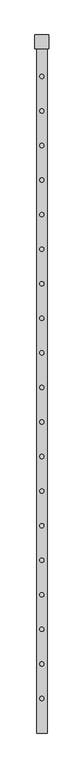
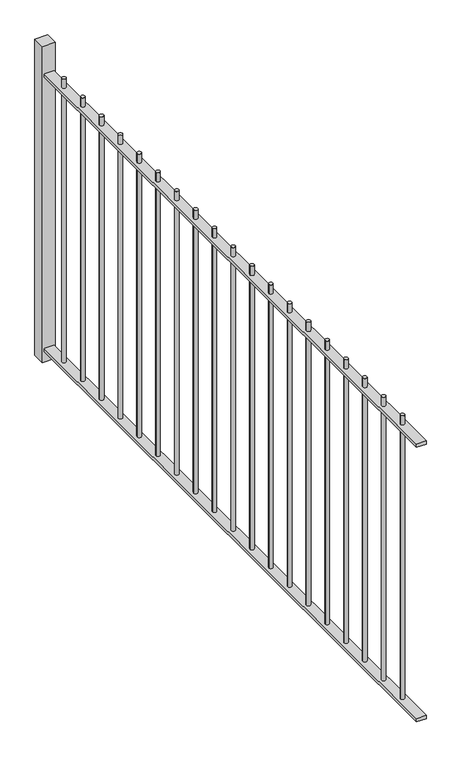
"""IFC4 building model written with IfcOpenShell, lengths in millimetres: railing geometry."""

from ifc_helpers import new_model, si_unit, point, frame, frame_2d, origin, place, context, project, spatial, polyline, circle_curve, trimmed, segment, composite_curve, outline, extrude, source, transform, mapped, element, save


def railing_16b95b7e(model_context):
    return source(origin(), model_context, "Body", "SweptSolid", [
        extrude(outline(polyline([(-6549.419961, -12811.1119119), (-6489.419961, -12811.1119119), (-6489.419961, -16811.1119119), (-6549.419961, -16811.1119119), (-6549.419961, -12811.1119119)])), frame((0.0, 0.0, -30.0), z_axis=(0.0, 0.0, 1.0), x_axis=(1.0, 0.0, 0.0)), (0.0, 0.0, 1.0), 20.0),
        extrude(outline(polyline([(-6549.419961, -12811.1119119), (-6489.419961, -12811.1119119), (-6489.419961, -16811.1119119), (-6549.419961, -16811.1119119), (-6549.419961, -12811.1119119)])), frame((0.0, 0.0, 1750.0), z_axis=(0.0, 0.0, 1.0), x_axis=(1.0, 0.0, 0.0)), (0.0, 0.0, 1.0), 20.0),
        extrude(outline(composite_curve([segment(trimmed(circle_curve(frame_2d((-6519.419961, -16611.1119119)), 12.5), [point((-6531.919961, -16611.1119119))], [point((-6506.919961, -16611.1119119))], False, "CARTESIAN"), True, "CONTINUOUS"), segment(trimmed(circle_curve(frame_2d((-6519.419961, -16611.1119119)), 12.5), [point((-6506.919961, -16611.1119119))], [point((-6531.919961, -16611.1119119))], False, "CARTESIAN"), True, "CONTINUOUS")], self_intersect=False)), frame((0.0, 0.0, -10.0), z_axis=(0.0, 0.0, 1.0), x_axis=(1.0, 0.0, 0.0)), (0.0, 0.0, 1.0), 1840.0),
        extrude(outline(composite_curve([segment(trimmed(circle_curve(frame_2d((-6519.419961, -16411.1119119)), 12.5), [point((-6531.919961, -16411.1119119))], [point((-6506.919961, -16411.1119119))], False, "CARTESIAN"), True, "CONTINUOUS"), segment(trimmed(circle_curve(frame_2d((-6519.419961, -16411.1119119)), 12.5), [point((-6506.919961, -16411.1119119))], [point((-6531.919961, -16411.1119119))], False, "CARTESIAN"), True, "CONTINUOUS")], self_intersect=False)), frame((0.0, 0.0, -10.0), z_axis=(0.0, 0.0, 1.0), x_axis=(1.0, 0.0, 0.0)), (0.0, 0.0, 1.0), 1840.0),
        extrude(outline(composite_curve([segment(trimmed(circle_curve(frame_2d((-6519.419961, -16211.1119119)), 12.5), [point((-6531.919961, -16211.1119119))], [point((-6506.919961, -16211.1119119))], False, "CARTESIAN"), True, "CONTINUOUS"), segment(trimmed(circle_curve(frame_2d((-6519.419961, -16211.1119119)), 12.5), [point((-6506.919961, -16211.1119119))], [point((-6531.919961, -16211.1119119))], False, "CARTESIAN"), True, "CONTINUOUS")], self_intersect=False)), frame((0.0, 0.0, -10.0), z_axis=(0.0, 0.0, 1.0), x_axis=(1.0, 0.0, 0.0)), (0.0, 0.0, 1.0), 1840.0),
        extrude(outline(composite_curve([segment(trimmed(circle_curve(frame_2d((-6519.419961, -16011.1119119)), 12.5), [point((-6531.919961, -16011.1119119))], [point((-6506.919961, -16011.1119119))], False, "CARTESIAN"), True, "CONTINUOUS"), segment(trimmed(circle_curve(frame_2d((-6519.419961, -16011.1119119)), 12.5), [point((-6506.919961, -16011.1119119))], [point((-6531.919961, -16011.1119119))], False, "CARTESIAN"), True, "CONTINUOUS")], self_intersect=False)), frame((0.0, 0.0, -10.0), z_axis=(0.0, 0.0, 1.0), x_axis=(1.0, 0.0, 0.0)), (0.0, 0.0, 1.0), 1840.0),
        extrude(outline(composite_curve([segment(trimmed(circle_curve(frame_2d((-6519.419961, -15811.1119119)), 12.5), [point((-6531.919961, -15811.1119119))], [point((-6506.919961, -15811.1119119))], False, "CARTESIAN"), True, "CONTINUOUS"), segment(trimmed(circle_curve(frame_2d((-6519.419961, -15811.1119119)), 12.5), [point((-6506.919961, -15811.1119119))], [point((-6531.919961, -15811.1119119))], False, "CARTESIAN"), True, "CONTINUOUS")], self_intersect=False)), frame((0.0, 0.0, -10.0), z_axis=(0.0, 0.0, 1.0), x_axis=(1.0, 0.0, 0.0)), (0.0, 0.0, 1.0), 1840.0),
        extrude(outline(composite_curve([segment(trimmed(circle_curve(frame_2d((-6519.419961, -15611.1119119)), 12.5), [point((-6531.919961, -15611.1119119))], [point((-6506.919961, -15611.1119119))], False, "CARTESIAN"), True, "CONTINUOUS"), segment(trimmed(circle_curve(frame_2d((-6519.419961, -15611.1119119)), 12.5), [point((-6506.919961, -15611.1119119))], [point((-6531.919961, -15611.1119119))], False, "CARTESIAN"), True, "CONTINUOUS")], self_intersect=False)), frame((0.0, 0.0, -10.0), z_axis=(0.0, 0.0, 1.0), x_axis=(1.0, 0.0, 0.0)), (0.0, 0.0, 1.0), 1840.0),
        extrude(outline(composite_curve([segment(trimmed(circle_curve(frame_2d((-6519.419961, -15411.1119119)), 12.5), [point((-6531.919961, -15411.1119119))], [point((-6506.919961, -15411.1119119))], False, "CARTESIAN"), True, "CONTINUOUS"), segment(trimmed(circle_curve(frame_2d((-6519.419961, -15411.1119119)), 12.5), [point((-6506.919961, -15411.1119119))], [point((-6531.919961, -15411.1119119))], False, "CARTESIAN"), True, "CONTINUOUS")], self_intersect=False)), frame((0.0, 0.0, -10.0), z_axis=(0.0, 0.0, 1.0), x_axis=(1.0, 0.0, 0.0)), (0.0, 0.0, 1.0), 1840.0),
        extrude(outline(composite_curve([segment(trimmed(circle_curve(frame_2d((-6519.419961, -15211.1119119)), 12.5), [point((-6531.919961, -15211.1119119))], [point((-6506.919961, -15211.1119119))], False, "CARTESIAN"), True, "CONTINUOUS"), segment(trimmed(circle_curve(frame_2d((-6519.419961, -15211.1119119)), 12.5), [point((-6506.919961, -15211.1119119))], [point((-6531.919961, -15211.1119119))], False, "CARTESIAN"), True, "CONTINUOUS")], self_intersect=False)), frame((0.0, 0.0, -10.0), z_axis=(0.0, 0.0, 1.0), x_axis=(1.0, 0.0, 0.0)), (0.0, 0.0, 1.0), 1840.0),
        extrude(outline(composite_curve([segment(trimmed(circle_curve(frame_2d((-6519.419961, -15011.1119119)), 12.5), [point((-6531.919961, -15011.1119119))], [point((-6506.919961, -15011.1119119))], False, "CARTESIAN"), True, "CONTINUOUS"), segment(trimmed(circle_curve(frame_2d((-6519.419961, -15011.1119119)), 12.5), [point((-6506.919961, -15011.1119119))], [point((-6531.919961, -15011.1119119))], False, "CARTESIAN"), True, "CONTINUOUS")], self_intersect=False)), frame((0.0, 0.0, -10.0), z_axis=(0.0, 0.0, 1.0), x_axis=(1.0, 0.0, 0.0)), (0.0, 0.0, 1.0), 1840.0),
        extrude(outline(composite_curve([segment(trimmed(circle_curve(frame_2d((-6519.419961, -14811.1119119)), 12.5), [point((-6531.919961, -14811.1119119))], [point((-6506.919961, -14811.1119119))], False, "CARTESIAN"), True, "CONTINUOUS"), segment(trimmed(circle_curve(frame_2d((-6519.419961, -14811.1119119)), 12.5), [point((-6506.919961, -14811.1119119))], [point((-6531.919961, -14811.1119119))], False, "CARTESIAN"), True, "CONTINUOUS")], self_intersect=False)), frame((0.0, 0.0, -10.0), z_axis=(0.0, 0.0, 1.0), x_axis=(1.0, 0.0, 0.0)), (0.0, 0.0, 1.0), 1840.0),
        extrude(outline(composite_curve([segment(trimmed(circle_curve(frame_2d((-6519.419961, -14611.1119119)), 12.5), [point((-6531.919961, -14611.1119119))], [point((-6506.919961, -14611.1119119))], False, "CARTESIAN"), True, "CONTINUOUS"), segment(trimmed(circle_curve(frame_2d((-6519.419961, -14611.1119119)), 12.5), [point((-6506.919961, -14611.1119119))], [point((-6531.919961, -14611.1119119))], False, "CARTESIAN"), True, "CONTINUOUS")], self_intersect=False)), frame((0.0, 0.0, -10.0), z_axis=(0.0, 0.0, 1.0), x_axis=(1.0, 0.0, 0.0)), (0.0, 0.0, 1.0), 1840.0),
        extrude(outline(composite_curve([segment(trimmed(circle_curve(frame_2d((-6519.419961, -14411.1119119)), 12.5), [point((-6531.919961, -14411.1119119))], [point((-6506.919961, -14411.1119119))], False, "CARTESIAN"), True, "CONTINUOUS"), segment(trimmed(circle_curve(frame_2d((-6519.419961, -14411.1119119)), 12.5), [point((-6506.919961, -14411.1119119))], [point((-6531.919961, -14411.1119119))], False, "CARTESIAN"), True, "CONTINUOUS")], self_intersect=False)), frame((0.0, 0.0, -10.0), z_axis=(0.0, 0.0, 1.0), x_axis=(1.0, 0.0, 0.0)), (0.0, 0.0, 1.0), 1840.0),
        extrude(outline(composite_curve([segment(trimmed(circle_curve(frame_2d((-6519.419961, -14211.1119119)), 12.5), [point((-6531.919961, -14211.1119119))], [point((-6506.919961, -14211.1119119))], False, "CARTESIAN"), True, "CONTINUOUS"), segment(trimmed(circle_curve(frame_2d((-6519.419961, -14211.1119119)), 12.5), [point((-6506.919961, -14211.1119119))], [point((-6531.919961, -14211.1119119))], False, "CARTESIAN"), True, "CONTINUOUS")], self_intersect=False)), frame((0.0, 0.0, -10.0), z_axis=(0.0, 0.0, 1.0), x_axis=(1.0, 0.0, 0.0)), (0.0, 0.0, 1.0), 1840.0),
        extrude(outline(composite_curve([segment(trimmed(circle_curve(frame_2d((-6519.419961, -14011.1119119)), 12.5), [point((-6531.919961, -14011.1119119))], [point((-6506.919961, -14011.1119119))], False, "CARTESIAN"), True, "CONTINUOUS"), segment(trimmed(circle_curve(frame_2d((-6519.419961, -14011.1119119)), 12.5), [point((-6506.919961, -14011.1119119))], [point((-6531.919961, -14011.1119119))], False, "CARTESIAN"), True, "CONTINUOUS")], self_intersect=False)), frame((0.0, 0.0, -10.0), z_axis=(0.0, 0.0, 1.0), x_axis=(1.0, 0.0, 0.0)), (0.0, 0.0, 1.0), 1840.0),
        extrude(outline(composite_curve([segment(trimmed(circle_curve(frame_2d((-6519.419961, -13811.1119119)), 12.5), [point((-6531.919961, -13811.1119119))], [point((-6506.919961, -13811.1119119))], False, "CARTESIAN"), True, "CONTINUOUS"), segment(trimmed(circle_curve(frame_2d((-6519.419961, -13811.1119119)), 12.5), [point((-6506.919961, -13811.1119119))], [point((-6531.919961, -13811.1119119))], False, "CARTESIAN"), True, "CONTINUOUS")], self_intersect=False)), frame((0.0, 0.0, -10.0), z_axis=(0.0, 0.0, 1.0), x_axis=(1.0, 0.0, 0.0)), (0.0, 0.0, 1.0), 1840.0),
        extrude(outline(composite_curve([segment(trimmed(circle_curve(frame_2d((-6519.419961, -13611.1119119)), 12.5), [point((-6531.919961, -13611.1119119))], [point((-6506.919961, -13611.1119119))], False, "CARTESIAN"), True, "CONTINUOUS"), segment(trimmed(circle_curve(frame_2d((-6519.419961, -13611.1119119)), 12.5), [point((-6506.919961, -13611.1119119))], [point((-6531.919961, -13611.1119119))], False, "CARTESIAN"), True, "CONTINUOUS")], self_intersect=False)), frame((0.0, 0.0, -10.0), z_axis=(0.0, 0.0, 1.0), x_axis=(1.0, 0.0, 0.0)), (0.0, 0.0, 1.0), 1840.0),
        extrude(outline(composite_curve([segment(trimmed(circle_curve(frame_2d((-6519.419961, -13411.1119119)), 12.5), [point((-6531.919961, -13411.1119119))], [point((-6506.919961, -13411.1119119))], False, "CARTESIAN"), True, "CONTINUOUS"), segment(trimmed(circle_curve(frame_2d((-6519.419961, -13411.1119119)), 12.5), [point((-6506.919961, -13411.1119119))], [point((-6531.919961, -13411.1119119))], False, "CARTESIAN"), True, "CONTINUOUS")], self_intersect=False)), frame((0.0, 0.0, -10.0), z_axis=(0.0, 0.0, 1.0), x_axis=(1.0, 0.0, 0.0)), (0.0, 0.0, 1.0), 1840.0),
        extrude(outline(composite_curve([segment(trimmed(circle_curve(frame_2d((-6519.419961, -13211.1119119)), 12.5), [point((-6531.919961, -13211.1119119))], [point((-6506.919961, -13211.1119119))], False, "CARTESIAN"), True, "CONTINUOUS"), segment(trimmed(circle_curve(frame_2d((-6519.419961, -13211.1119119)), 12.5), [point((-6506.919961, -13211.1119119))], [point((-6531.919961, -13211.1119119))], False, "CARTESIAN"), True, "CONTINUOUS")], self_intersect=False)), frame((0.0, 0.0, -10.0), z_axis=(0.0, 0.0, 1.0), x_axis=(1.0, 0.0, 0.0)), (0.0, 0.0, 1.0), 1840.0),
        extrude(outline(composite_curve([segment(trimmed(circle_curve(frame_2d((-6519.419961, -13011.1119119)), 12.5), [point((-6531.919961, -13011.1119119))], [point((-6506.919961, -13011.1119119))], False, "CARTESIAN"), True, "CONTINUOUS"), segment(trimmed(circle_curve(frame_2d((-6519.419961, -13011.1119119)), 12.5), [point((-6506.919961, -13011.1119119))], [point((-6531.919961, -13011.1119119))], False, "CARTESIAN"), True, "CONTINUOUS")], self_intersect=False)), frame((0.0, 0.0, -10.0), z_axis=(0.0, 0.0, 1.0), x_axis=(1.0, 0.0, 0.0)), (0.0, 0.0, 1.0), 1840.0),
        extrude(outline(polyline([(-6479.419961, -12771.1119119), (-6479.419961, -12851.1119119), (-6559.419961, -12851.1119119), (-6559.419961, -12771.1119119), (-6479.419961, -12771.1119119)])), frame((0.0, 0.0, -100.0), z_axis=(0.0, 0.0, 1.0), x_axis=(1.0, 0.0, 0.0)), (0.0, 0.0, 1.0), 2050.0),
    ])


if __name__ == "__main__":
    model = new_model("IFC4")
    model_context = context("Model", 3, world=origin())
    ifc_project = project(units=[si_unit("LENGTHUNIT", "METRE", prefix="MILLI")], contexts=[model_context])
    site = spatial("IfcSite", under=ifc_project)
    building = spatial("IfcBuilding", under=site)
    placement = place(None, origin())
    railing_shape = railing_16b95b7e(model_context)
    element("IfcRailing", 1, at=placement, inside=building, context=model_context, shape_type="MappedRepresentation", body=[
        mapped(railing_shape, transform((0.0, 0.0, 0.0), x_axis=(1.0, 0.0, 0.0), y_axis=(0.0, 1.0, 0.0), z_axis=(0.0, 0.0, 1.0))),
    ])
    save(model, "model.ifc")

# Revit data of these elements
# Element 1 (IfcRailing)
#   Materials on its faces: "NLRS_h2_staal_generiek zwart_gen_rsf", "NLRS_h2_staal_gen_rsf"
# Materials
#   "NLRS_h2_staal_generiek zwart_gen_rsf": class "Metal", colour RGB 189 187 185, transparency 0, Manufacturer = "RevitGG", URL = "www.revitgg.nl", Description = "Staal, generiek materiaal", Cost = 0
#   "NLRS_h2_staal_gen_rsf": class "H - Metaal", colour RGB 189 187 185, transparency 0, Keynote = "h2", Model = "generiek", Manufacturer = "Revit Standards Foundation", URL = "www.revitstandards.org", Description = "staal", Cost = 0
